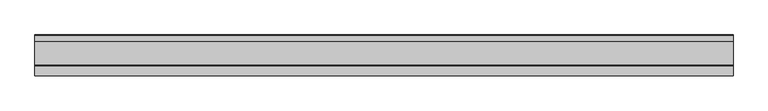
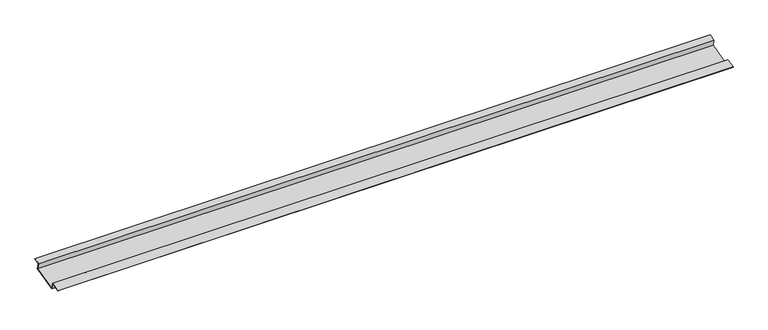
"""IFC4 building model written with IfcOpenShell, lengths in millimetres: proxy geometry, Soffit003 4791 : Soffit003 4791."""

from ifc_helpers import new_model, si_unit, frame, origin, place, context, project, spatial, polyline, outline, extrude, source, transform, mapped, element, save


def generic_models_57078732(model_context):
    return source(origin(), model_context, "Body", "SweptSolid", [
        extrude(outline(polyline([(-5244.0236011, 42427.9124632), (-5239.3852349, 42409.3953515), (-5313.3015493, 42390.8799942), (-5317.9399151, 42409.4022563), (-5343.409089, 42403.024237), (-5343.7175976, 42404.2561958), (-5317.0164648, 42410.9427236), (-5312.3781193, 42392.4205423), (-5240.9257627, 42410.3187007), (-5245.5641492, 42428.8358932), (-5227.0077672, 42433.4828034), (-5226.6992587, 42432.2508446), (-5244.0236011, 42427.9124632)])), frame((12382.7678845, 0.0, 0.0), z_axis=(1.0, 0.0, 0.0), x_axis=(0.0, 1.0, 0.0)), (0.0, 0.0, 1.0), 2000.25),
    ])


if __name__ == "__main__":
    model = new_model("IFC4")
    model_context = context("Model", 3, world=origin())
    ifc_project = project(units=[si_unit("LENGTHUNIT", "METRE", prefix="MILLI")], contexts=[model_context])
    site = spatial("IfcSite", under=ifc_project)
    building = spatial("IfcBuilding", under=site)
    placement = place(None, origin())
    generic_models_shape = generic_models_57078732(model_context)
    element("IfcBuildingElementProxy", 1, Name="Soffit003 4791 : Soffit003 4791", ObjectType="Soffit003 4791 : Soffit003 4791", at=placement, inside=building, context=model_context, shape_type="MappedRepresentation", body=[
        mapped(generic_models_shape, transform((0.0, 0.0, 0.0), x_axis=(1.0, 0.0, 0.0), y_axis=(0.0, 1.0, 0.0), z_axis=(0.0, 0.0, 1.0))),
    ])
    save(model, "model.ifc")

# Revit data of these elements
# Type "Soffit003 4791 : Soffit003 4791"
#   NameOverride = "Soffit003"
# Element 1 (IfcBuildingElementProxy, "Soffit003 4791 : Soffit003 4791")
#   Materials on its faces: "16 GA. COPPER SOFFIT VENT - VERIFY W/ ARCHITECT ON LOCATION"
# Materials
#   "16 GA. COPPER SOFFIT VENT - VERIFY W/ ARCHITECT ON LOCATION": class "Unassigned", colour RGB 85 255 127, transparency 0
